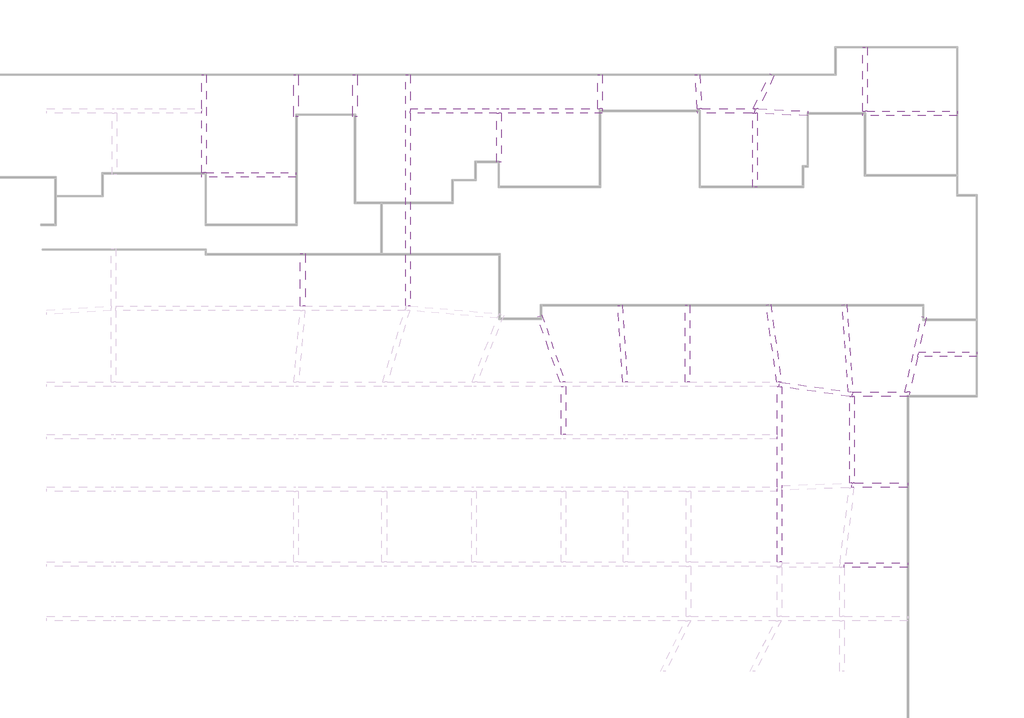
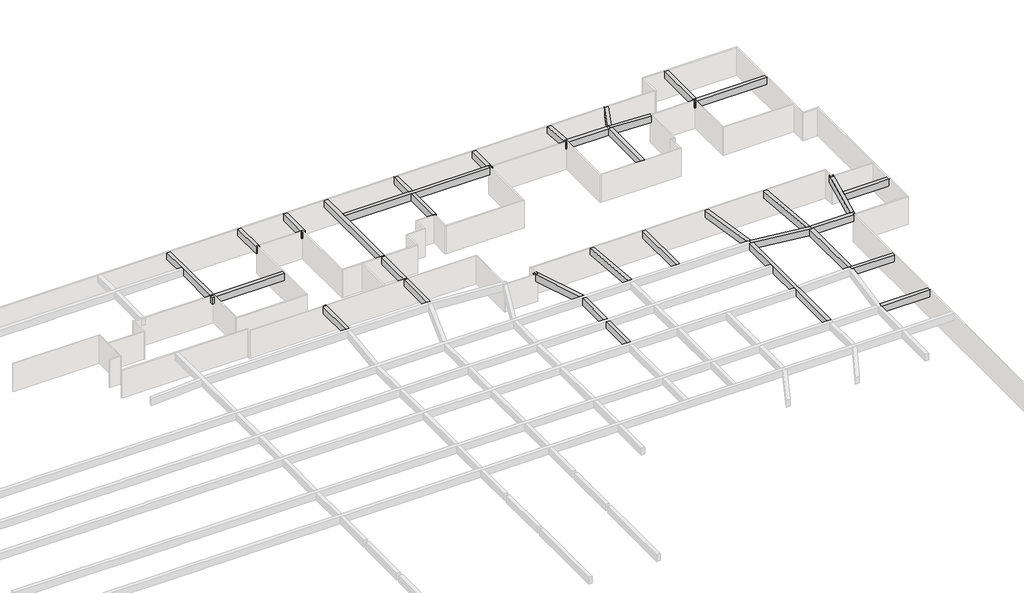
# One storey, part 45 of 45: 30 beams.
"""IFC4 building model written with IfcOpenShell, lengths in millimetres."""

import ifcopenshell
import ifcopenshell.guid

model = None  # the IFC model being written
_history = None  # IfcOwnerHistory: only IFC2X3 demands one
_inside = {}  # id of a spatial element -> (the spatial element, [elements in it])
_under = {}  # id of a project, library or spatial element -> (it, [spatial elements below it])
_declared = {}  # id of a project -> (the project, [libraries it declares])
_typed = {}  # id of a type object -> (the type object, [elements of that type])
_made_of = {}  # id of a material, layer set ... -> (it, [elements and type objects made of it])


def new_model(schema):
    """Start an empty IFC model of exactly this schema.

    Asked for "IFC4X3", IfcOpenShell would pick the latest addendum, in which some entities
    have other attributes; the version numbers below select the first issue.
    IFC2X3 requires an IfcOwnerHistory on every rooted entity: one is made here for all.
    """
    global model, _history
    if schema == "IFC4X3":
        model = ifcopenshell.file(schema_version=(4, 3, 0, 0))
    else:
        model = ifcopenshell.file(schema=schema)
    _inside.clear()
    _under.clear()
    _declared.clear()
    _typed.clear()
    _made_of.clear()
    _history = None
    if model.schema == "IFC2X3":
        org = make("IfcOrganization", Name="unknown")
        user = make(
            "IfcPersonAndOrganization",
            ThePerson=make("IfcPerson", FamilyName="unknown"),
            TheOrganization=org,
        )
        app = make(
            "IfcApplication",
            ApplicationDeveloper=org,
            Version="unknown",
            ApplicationFullName="unknown",
            ApplicationIdentifier="unknown",
        )
        _history = make(
            "IfcOwnerHistory",
            OwningUser=user,
            OwningApplication=app,
            ChangeAction="ADDED",
            CreationDate=0,
        )
    return model


def make(cls, **values):
    """One entity of the class cls with the attributes given. An attribute that is None is left unset."""
    return model.create_entity(
        cls, **{name: value for name, value in values.items() if value is not None}
    )


def rooted(cls, **values):
    """An entity with a GlobalId (a new one), such as an element, a storey or a relation."""
    return make(cls, GlobalId=ifcopenshell.guid.new(), OwnerHistory=_history, **values)


def si_unit(unit_type, name, prefix=None):
    """IfcSIUnit, for example si_unit("LENGTHUNIT", "METRE", prefix="MILLI")."""
    return make("IfcSIUnit", UnitType=unit_type, Prefix=prefix, Name=name)


def assignment(units):
    """IfcUnitAssignment: the units of a project."""
    return None if units is None else make("IfcUnitAssignment", Units=units)


def point(xyz):
    """IfcCartesianPoint."""
    return None if xyz is None else make("IfcCartesianPoint", Coordinates=xyz)


def direction(xyz):
    """IfcDirection."""
    return None if xyz is None else make("IfcDirection", DirectionRatios=xyz)


def frame(location, z_axis=None, x_axis=None):
    """IfcAxis2Placement3D, a coordinate frame: its origin and axes. An axis left out is left unset."""
    return make(
        "IfcAxis2Placement3D",
        Location=point(location),
        Axis=direction(z_axis),
        RefDirection=direction(x_axis),
    )


def origin():
    """The frame at (0, 0, 0) with its axes left unset."""
    return frame((0.0, 0.0, 0.0))


def place(relative_to, where):
    """IfcLocalPlacement: puts the frame where relative to a parent placement (None: the world)."""
    return make(
        "IfcLocalPlacement", PlacementRelTo=relative_to, RelativePlacement=where
    )


def context(
    kind, dimensions, precision=None, world=None, true_north=None, identifier=None
):
    """IfcGeometricRepresentationContext, for example the 3D "Model" context."""
    return make(
        "IfcGeometricRepresentationContext",
        ContextIdentifier=identifier,
        ContextType=kind,
        CoordinateSpaceDimension=dimensions,
        Precision=precision,
        WorldCoordinateSystem=world,
        TrueNorth=true_north,
    )


def project(units=None, contexts=None):
    """IfcProject with its units and contexts."""
    return rooted(
        "IfcProject",
        Name="project",
        RepresentationContexts=contexts,
        UnitsInContext=assignment(units),
    )


def spatial(cls, under=None, at=None, **own):
    """A site, building, storey or space (cls), placed at a placement, below another one or the project."""
    s = rooted(cls, ObjectPlacement=at, **own)
    if under is not None:
        _under.setdefault(under.id(), (under, []))[1].append(s)
    return s


def polyline(points):
    """IfcPolyline through the points."""
    return make("IfcPolyline", Points=[point(p) for p in points])


def outline(outer, holes=None, kind="AREA"):
    """IfcArbitraryClosedProfileDef: a profile drawn as a closed curve; with holes, ...WithVoids."""
    if holes is None:
        return make("IfcArbitraryClosedProfileDef", ProfileType=kind, OuterCurve=outer)
    return make(
        "IfcArbitraryProfileDefWithVoids",
        ProfileType=kind,
        OuterCurve=outer,
        InnerCurves=holes,
    )


def extrude(swept, where, along, depth):
    """IfcExtrudedAreaSolid: the profile swept, set in the frame where, extruded along a direction by depth."""
    return make(
        "IfcExtrudedAreaSolid",
        SweptArea=swept,
        Position=where,
        ExtrudedDirection=direction(along),
        Depth=depth,
    )


def faces_of(points, faces, orient=None, outer=None):
    """IfcFace entities. A face is a list of loops; a loop is a list of indices into points, from 0.

    orient and outer hold one flag for each loop. By default every Orientation is true, the
    first loop of a face is its IfcFaceOuterBound and the others are IfcFaceBound.
    """
    made = []
    for i, loops in enumerate(faces):
        bounds = []
        for j, loop in enumerate(loops):
            is_outer = j == 0 if outer is None else outer[i][j]
            bounds.append(
                make(
                    "IfcFaceOuterBound" if is_outer else "IfcFaceBound",
                    Bound=make("IfcPolyLoop", Polygon=[points[k] for k in loop]),
                    Orientation=True if orient is None else orient[i][j],
                )
            )
        made.append(make("IfcFace", Bounds=bounds))
    return made


def faceted_brep(points, faces, orient=None, outer=None, voids=None):
    """IfcFacetedBrep: a solid bounded by flat faces; with voids (closed shells), ...WithVoids."""
    shared = [point(p) for p in points]
    hull = make("IfcClosedShell", CfsFaces=faces_of(shared, faces, orient, outer))
    if voids is None:
        return make("IfcFacetedBrep", Outer=hull)
    return make(
        "IfcFacetedBrepWithVoids",
        Outer=hull,
        Voids=[
            make(cls, CfsFaces=faces_of(shared, fs, o, b)) for cls, fs, o, b in voids
        ],
    )


def shape(context_of_items, identifier, shape_type, items):
    """IfcShapeRepresentation: the items that make up one representation, for example the "Body"."""
    return make(
        "IfcShapeRepresentation",
        ContextOfItems=context_of_items,
        RepresentationIdentifier=identifier,
        RepresentationType=shape_type,
        Items=items,
    )


def source(mapping_origin, context_of_items, identifier, shape_type, items):
    """IfcRepresentationMap: a shape defined once, which mapped items show again and again."""
    return make(
        "IfcRepresentationMap",
        MappingOrigin=mapping_origin,
        MappedRepresentation=shape(context_of_items, identifier, shape_type, items),
    )


def transform(
    local_origin,
    x_axis=None,
    y_axis=None,
    z_axis=None,
    scale=None,
    scale2=None,
    scale3=None,
    uniform=True,
):
    """IfcCartesianTransformationOperator3D, or its non-uniform kind. x_axis, y_axis, z_axis: its Axis1, 2, 3."""
    if uniform:
        return make(
            "IfcCartesianTransformationOperator3D",
            Axis1=direction(x_axis),
            Axis2=direction(y_axis),
            LocalOrigin=point(local_origin),
            Scale=scale,
            Axis3=direction(z_axis),
        )
    return make(
        "IfcCartesianTransformationOperator3DnonUniform",
        Axis1=direction(x_axis),
        Axis2=direction(y_axis),
        LocalOrigin=point(local_origin),
        Scale=scale,
        Axis3=direction(z_axis),
        Scale2=scale2,
        Scale3=scale3,
    )


def mapped(mapping_source, mapping_target):
    """IfcMappedItem: shows the shape of a source again, moved by a transform."""
    return make(
        "IfcMappedItem", MappingSource=mapping_source, MappingTarget=mapping_target
    )


def made_of(thing, what):
    """Note that an element or type object is made of a material, layer set ...; save() writes the relation."""
    if what is not None:
        _made_of.setdefault(what.id(), (what, []))[1].append(thing)
    return thing


def element(
    cls,
    number,
    at=None,
    inside=None,
    cuts=None,
    type_object=None,
    material=None,
    context=None,
    identifier="Body",
    shape_type=None,
    held_by="IfcProductDefinitionShape",
    body=None,
    shapes=None,
    **own,
):
    """One element of the class cls, such as IfcWall. Its Tag is "e" and its number.

    at: its placement. inside: the storey or other place that contains it. cuts: it is an
    opening in that element (IfcRelVoidsElement). A single representation is given by context,
    identifier, shape_type and body (its items); several are given by shapes. held_by: the class
    of the entity that holds the representations. save() writes the other relations.
    """
    e = rooted(cls, Tag="e%d" % number, ObjectPlacement=at, **own)
    if body is not None:
        shapes = [shape(context, identifier, shape_type, body)]
    if shapes is not None:
        e.Representation = make(held_by, Representations=shapes)
    if inside is not None:
        _inside.setdefault(inside.id(), (inside, []))[1].append(e)
    if cuts is not None:
        rooted(
            "IfcRelVoidsElement", RelatingBuildingElement=cuts, RelatedOpeningElement=e
        )
    if type_object is not None:
        _typed.setdefault(type_object.id(), (type_object, []))[1].append(e)
    return made_of(e, material)


def aggregate(whole, parts):
    """IfcRelAggregates: a whole, such as a stair, and the parts it consists of."""
    return rooted("IfcRelAggregates", RelatingObject=whole, RelatedObjects=parts)


def save(model, path):
    """Write the relations noted so far, then the file.

    IfcRelAggregates (storeys below a building ...), IfcRelContainedInSpatialStructure (elements
    in a storey), IfcRelDefinesByType, IfcRelAssociatesMaterial and IfcRelDeclares: one each for
    every whole, place, type object, material and project.
    """
    for whole, parts in _under.values():
        aggregate(whole, parts)
    for where, things in _inside.values():
        rooted(
            "IfcRelContainedInSpatialStructure",
            RelatedElements=things,
            RelatingStructure=where,
        )
    for kind, things in _typed.values():
        rooted("IfcRelDefinesByType", RelatedObjects=things, RelatingType=kind)
    for what, things in _made_of.values():
        rooted("IfcRelAssociatesMaterial", RelatedObjects=things, RelatingMaterial=what)
    for by, libraries in _declared.values():
        rooted("IfcRelDeclares", RelatingContext=by, RelatedDefinitions=libraries)
    model.write(path)


def kl_beam_c459b6d2(model_context):
    return source(origin(), model_context, "Body", "SweptSolid", [
        extrude(outline(polyline([(1817.0, 200.0), (1817.0, -200.0), (-1817.0, -200.0), (-1817.0, 200.0), (1817.0, 200.0)])), frame((0.0, 0.0, -400.0), z_axis=(0.0, 0.0, 1.0), x_axis=(1.0, 0.0, 0.0)), (0.0, 0.0, 1.0), 800.0),
    ])


def kl_beam_000e6cef(model_context):
    return source(origin(), model_context, "Body", "SweptSolid", [
        extrude(outline(polyline([(1827.5, 200.0), (1827.5, -200.0), (-1827.5, -200.0), (-1827.5, 200.0), (1827.5, 200.0)])), frame((0.0, 0.0, -400.0), z_axis=(0.0, 0.0, 1.0), x_axis=(1.0, 0.0, 0.0)), (0.0, 0.0, 1.0), 800.0),
    ])


model = new_model("IFC4")

# Units and contexts
model_context = context("Model", 3, world=origin())
ifc_project = project(units=[si_unit("LENGTHUNIT", "METRE", prefix="MILLI")], contexts=[model_context])

# Site, building, storey
site = spatial("IfcSite", under=ifc_project)
building = spatial("IfcBuilding", under=site)
storey = spatial("IfcBuildingStorey", under=building, Name="户型图", Elevation=0.0)

# Beams
placement = place(None, origin())
element("IfcBeam", 1, ObjectType="混凝土 - 矩形梁 : KL_beam", at=placement, inside=storey, context=model_context, shape_type="SweptSolid", body=[
    extrude(outline(polyline([(10558.170888, 195578.568213), (10958.170888, 195578.568213), (10958.170888, 191034.1392013), (10558.170888, 191034.1392013), (10558.170888, 195578.568213)])), frame((0.0, 0.0, 2500.0), z_axis=(0.0, 0.0, 1.0), x_axis=(1.0, 0.0, 0.0)), (0.0, 0.0, 1.0), 800.0),
])
element("IfcBeam", 2, ObjectType="混凝土 - 矩形梁 : KL_beam", at=placement, inside=storey, context=model_context, shape_type="SweptSolid", body=[
    extrude(outline(polyline([(38177.3384091, 191063.5546545), (38576.3640292, 191091.457244), (39044.6739052, 184394.3140025), (38643.697146, 184394.3140025), (38177.3384091, 191063.5546545)])), frame((0.0, 0.0, 2500.0), z_axis=(0.0, 0.0, 1.0), x_axis=(1.0, 0.0, 0.0)), (0.0, 0.0, 1.0), 800.0),
])
element("IfcBeam", 3, ObjectType="混凝土 - 矩形梁 : KL_beam", at=placement, inside=storey, context=model_context, shape_type="SweptSolid", body=[
    extrude(outline(polyline([(44058.170888, 191094.3140025), (44458.170888, 191094.3140025), (44458.170888, 184394.3140025), (44058.170888, 184394.3140025), (44058.170888, 191094.3140025)])), frame((0.0, 0.0, 2500.0), z_axis=(0.0, 0.0, 1.0), x_axis=(1.0, 0.0, 0.0)), (0.0, 0.0, 1.0), 800.0),
])
element("IfcBeam", 4, ObjectType="混凝土 - 矩形梁 : KL_beam", at=placement, inside=storey, context=model_context, shape_type="Brep", body=[
    faceted_brep([(58656.8908977, 183499.9137112, 3300.0), (58251.9343991, 183556.8266355, 3300.0), (52455.9955059, 184371.3927255, 3300.0), (52292.9021454, 184394.3140025, 3300.0), (52264.9314206, 183994.3140025, 3300.0), (52492.6053307, 183962.3165211, 3300.0), (58384.2248716, 183134.3033931, 3300.0), (58601.2216573, 183103.8064837, 3300.0), (58604.1159054, 183124.4001284, 3300.0), (52264.9314206, 183994.3140025, 2500.0), (52492.6053307, 183962.3165211, 2500.0), (58384.2248716, 183134.3033931, 2500.0), (58601.2216573, 183103.8064837, 2500.0), (52292.9021454, 184394.3140025, 2500.0), (52455.9955059, 184371.3927255, 2500.0), (58251.9343991, 183556.8266355, 2500.0), (58656.8908977, 183499.9137112, 2500.0), (58604.1159054, 183124.4001284, 2500.0)], [[[0, 1, 2, 3, 4, 5, 6, 7, 8]], [[7, 6, 5, 4, 9, 10, 11, 12]], [[12, 11, 10, 9, 13, 14, 15, 16, 17]], [[3, 2, 1, 0, 16, 15, 14, 13]], [[3, 13, 9, 4]], [[0, 8, 7, 12, 17, 16]]]),
])
element("IfcBeam", 5, ObjectType="混凝土 - 矩形梁 : KL_beam", at=placement, inside=storey, context=model_context, shape_type="SweptSolid", body=[
    extrude(outline(polyline([(51106.6514625, 191098.3558635), (51502.75869, 191154.0251039), (52455.9955059, 184371.3927255), (52292.9021454, 184394.3140025), (52048.8431015, 184394.3140025), (51106.6514625, 191098.3558635)])), frame((0.0, 0.0, 2500.0), z_axis=(0.0, 0.0, 1.0), x_axis=(1.0, 0.0, 0.0)), (0.0, 0.0, 1.0), 800.0),
])
element("IfcBeam", 6, ObjectType="混凝土 - 矩形梁 : KL_beam", at=placement, inside=storey, context=model_context, shape_type="Brep", body=[
    faceted_brep([(58122.1746543, 191146.7122502, 3300.0), (58122.1746543, 191146.7122502, 2500.0), (57723.1490342, 191118.8096607, 2500.0), (57723.1490342, 191118.8096607, 3300.0), (58251.9343991, 183556.8266355, 3300.0), (58656.8908977, 183499.9137112, 3300.0), (58655.1786406, 183524.4001284, 3300.0), (58251.9343991, 183556.8266355, 2500.0), (58655.1786406, 183524.4001284, 2500.0), (58656.8908977, 183499.9137112, 2500.0)], [[[0, 1, 2, 3]], [[0, 3, 4, 5, 6]], [[3, 2, 7, 4]], [[2, 1, 8, 9, 7]], [[1, 0, 6, 5, 9, 8]], [[5, 4, 7, 9]]]),
])
element("IfcBeam", 7, ObjectType="混凝土 - 矩形梁 : KL_beam", at=placement, inside=storey, context=model_context, shape_type="Brep", body=[
    faceted_brep([(58656.8908977, 183499.9137112, 3300.0), (58604.1159054, 183124.4001284, 3300.0), (58784.2248716, 183124.4001284, 3300.0), (63529.491463, 183124.4001284, 3300.0), (63617.407341, 183524.4001284, 3300.0), (63207.8597838, 183524.4001284, 3300.0), (58655.1786406, 183524.4001284, 3300.0), (58604.1159054, 183124.4001284, 2500.0), (58784.2248716, 183124.4001284, 2500.0), (63529.491463, 183124.4001284, 2500.0), (58656.8908977, 183499.9137112, 2500.0), (58655.1786406, 183524.4001284, 2500.0), (63207.8597838, 183524.4001284, 2500.0), (63617.407341, 183524.4001284, 2500.0)], [[[0, 1, 2, 3, 4, 5, 6]], [[1, 7, 8, 9, 3, 2]], [[7, 10, 11, 12, 13, 9, 8]], [[4, 13, 12, 11, 6, 5]], [[1, 0, 10, 7]], [[0, 6, 11, 10]], [[4, 3, 9, 13]]]),
])
element("IfcBeam", 8, ObjectType="混凝土 - 矩形梁 : KL_beam", at=placement, inside=storey, context=model_context, shape_type="Brep", body=[
    faceted_brep([(65041.3670071, 190003.1373024, 3300.0), (65041.3670071, 190003.1373024, 2500.0), (64650.6919873, 190089.0036458, 2500.0), (64650.6919873, 190089.0036458, 3300.0), (63207.8597838, 183524.4001284, 3300.0), (63617.407341, 183524.4001284, 3300.0), (64298.4480041, 186623.0015609, 3300.0), (64386.363882, 187023.0015609, 3300.0), (63207.8597838, 183524.4001284, 2500.0), (64386.363882, 187023.0015609, 2500.0), (64298.4480041, 186623.0015609, 2500.0), (63617.407341, 183524.4001284, 2500.0)], [[[0, 1, 2, 3]], [[0, 3, 4, 5, 6, 7]], [[3, 2, 8, 4]], [[2, 1, 9, 10, 11, 8]], [[1, 0, 7, 6, 5, 11, 10, 9]], [[5, 4, 8, 11]]]),
])
element("IfcBeam", 9, ObjectType="混凝土 - 矩形梁 : KL_beam", at=placement, inside=storey, context=model_context, shape_type="SweptSolid", body=[
    extrude(outline(polyline([(69459.055254, 187023.0015609), (69459.055254, 186623.0015609), (64298.4480041, 186623.0015609), (64386.363882, 187023.0015609), (69459.055254, 187023.0015609)])), frame((0.0, 0.0, 2500.0), z_axis=(0.0, 0.0, 1.0), x_axis=(1.0, 0.0, 0.0)), (0.0, 0.0, 1.0), 800.0),
])
element("IfcBeam", 10, ObjectType="混凝土 - 矩形梁 : KL_beam", at=placement, inside=storey, context=model_context, shape_type="SweptSolid", body=[
    extrude(outline(polyline([(33258.170888, 183994.3140025), (33658.170888, 183994.3140025), (33658.170888, 179811.4368869), (33258.170888, 179811.4368869), (33258.170888, 183994.3140025)])), frame((0.0, 0.0, 2500.0), z_axis=(0.0, 0.0, 1.0), x_axis=(1.0, 0.0, 0.0)), (0.0, 0.0, 1.0), 800.0),
    extrude(outline(polyline([(33658.170888, 175259.2955299), (33258.170888, 175259.2955299), (33258.170888, 179411.4368869), (33658.170888, 179411.4368869), (33658.170888, 175259.2955299)])), frame((0.0, 0.0, 2500.0), z_axis=(0.0, 0.0, 1.0), x_axis=(1.0, 0.0, 0.0)), (0.0, 0.0, 1.0), 800.0),
])
element("IfcBeam", 11, ObjectType="混凝土 - 矩形梁 : KL_beam", at=placement, inside=storey, context=model_context, shape_type="SweptSolid", body=[
    extrude(outline(polyline([(31217.9877998, 190085.9673979), (31596.19523, 190216.1946597), (33600.8295016, 184394.3140025), (33177.7812291, 184394.3140025), (31217.9877998, 190085.9673979)])), frame((0.0, 0.0, 2500.0), z_axis=(0.0, 0.0, 1.0), x_axis=(1.0, 0.0, 0.0)), (0.0, 0.0, 1.0), 800.0),
])
element("IfcBeam", 12, ObjectType="混凝土 - 矩形梁 : KL_beam", at=placement, inside=storey, context=model_context, shape_type="Brep", body=[
    faceted_brep([(19735.6474887, 211171.5634374, 3300.0), (20135.6474887, 211171.5634374, 3300.0), (20135.6474887, 211171.5634374, 2500.0), (19735.6474887, 211171.5634374, 2500.0), (19735.6474887, 191052.4009015, 3300.0), (20135.6474887, 191017.4054361, 3300.0), (20135.6474887, 207811.9876735, 3300.0), (20135.6474887, 208211.9876735, 3300.0), (20135.6474887, 191017.4054361, 2500.0), (20135.6474887, 207811.9876735, 2500.0), (20135.6474887, 208211.9876735, 2500.0), (19735.6474887, 191052.4009015, 2500.0)], [[[0, 1, 2, 3]], [[1, 0, 4, 5, 6, 7]], [[2, 1, 7, 6, 5, 8, 9, 10]], [[3, 2, 10, 9, 8, 11]], [[0, 3, 11, 4]], [[5, 4, 11, 8]]]),
])
element("IfcBeam", 13, ObjectType="混凝土 - 矩形梁 : KL_beam", at=placement, inside=storey, context=model_context, shape_type="Brep", body=[
    faceted_brep([(36835.6474887, 207811.9876735, 3300.0), (36835.6474887, 208211.9876735, 3300.0), (36435.6474887, 208211.9876735, 3300.0), (28035.6474887, 208211.9876735, 3300.0), (27635.6474887, 208211.9876735, 3300.0), (20135.6474887, 208211.9876735, 3300.0), (20135.6474887, 207811.9876735, 3300.0), (27635.6474887, 207811.9876735, 3300.0), (28035.6474887, 207811.9876735, 3300.0), (36835.6474887, 207811.9876735, 2500.0), (20135.6474887, 207811.9876735, 2500.0), (27635.6474887, 207811.9876735, 2500.0), (28035.6474887, 207811.9876735, 2500.0), (36835.6474887, 208211.9876735, 2500.0), (20135.6474887, 208211.9876735, 2500.0), (27635.6474887, 208211.9876735, 2500.0), (28035.6474887, 208211.9876735, 2500.0), (36435.6474887, 208211.9876735, 2500.0)], [[[0, 1, 2, 3, 4, 5, 6, 7, 8]], [[9, 0, 8, 7, 6, 10, 11, 12]], [[13, 9, 12, 11, 10, 14, 15, 16, 17]], [[1, 13, 17, 16, 15, 14, 5, 4, 3, 2]], [[6, 5, 14, 10]], [[1, 0, 9, 13]]]),
])
element("IfcBeam", 14, ObjectType="混凝土 - 矩形梁 : KL_beam", at=placement, inside=storey, context=model_context, shape_type="SweptSolid", body=[
    extrude(outline(polyline([(36435.6474887, 211171.9876735), (36835.6474887, 211171.9876735), (36835.6474887, 208211.9876735), (36435.6474887, 208211.9876735), (36435.6474887, 211171.9876735)])), frame((0.0, 0.0, 2500.0), z_axis=(0.0, 0.0, 1.0), x_axis=(1.0, 0.0, 0.0)), (0.0, 0.0, 1.0), 800.0),
])
element("IfcBeam", 15, ObjectType="混凝土 - 矩形梁 : KL_beam", at=placement, inside=storey, context=model_context, shape_type="SweptSolid", body=[
    extrude(outline(polyline([(28035.6474887, 203571.9876735), (27635.6474887, 203571.9876735), (27635.6474887, 207811.9876735), (28035.6474887, 207811.9876735), (28035.6474887, 203571.9876735)])), frame((0.0, 0.0, 2500.0), z_axis=(0.0, 0.0, 1.0), x_axis=(1.0, 0.0, 0.0)), (0.0, 0.0, 1.0), 800.0),
    extrude(outline(polyline([(27635.6474887, 211171.9876735), (28035.6474887, 211171.9876735), (28035.6474887, 208211.9876735), (27635.6474887, 208211.9876735), (27635.6474887, 211171.9876735)])), frame((0.0, 0.0, 2500.0), z_axis=(0.0, 0.0, 1.0), x_axis=(1.0, 0.0, 0.0)), (0.0, 0.0, 1.0), 800.0),
])
element("IfcBeam", 16, ObjectType="混凝土 - 矩形梁 : KL_beam", at=placement, inside=storey, context=model_context, shape_type="Brep", body=[
    faceted_brep([(10170.4764011, 202651.2886433, 3300.0), (10170.4764011, 202251.2886433, 3300.0), (10170.4764011, 202251.2886433, 2500.0), (10170.4764011, 202651.2886433, 2500.0), (2351.1462183, 202651.2886433, 3300.0), (1951.1462183, 202651.2886433, 3300.0), (1951.1462183, 202251.2886433, 3300.0), (1951.1462183, 202251.2886433, 2500.0), (1951.1462183, 202651.2886433, 2500.0), (2351.1462183, 202651.2886433, 2500.0)], [[[0, 1, 2, 3]], [[1, 0, 4, 5, 6]], [[2, 1, 6, 7]], [[3, 2, 7, 8, 9]], [[0, 3, 9, 8, 5, 4]], [[6, 5, 8, 7]]]),
])
element("IfcBeam", 17, ObjectType="混凝土 - 矩形梁 : KL_beam", at=placement, inside=storey, context=model_context, shape_type="Brep", body=[
    faceted_brep([(1951.1462183, 211171.6381584, 3300.0), (2351.1462183, 211171.6381584, 3300.0), (2351.1462183, 211171.6381584, 2500.0), (1951.1462183, 211171.6381584, 2500.0), (1951.1462183, 208211.9876735, 3300.0), (1951.1462183, 207811.9876735, 3300.0), (1951.1462183, 202651.2886433, 3300.0), (2351.1462183, 202651.2886433, 3300.0), (2351.1462183, 202651.2886433, 2500.0), (1951.1462183, 202651.2886433, 2500.0), (1951.1462183, 207811.9876735, 2500.0), (1951.1462183, 208211.9876735, 2500.0)], [[[0, 1, 2, 3]], [[1, 0, 4, 5, 6, 7]], [[2, 1, 7, 8]], [[3, 2, 8, 9, 10, 11]], [[0, 3, 11, 10, 9, 6, 5, 4]], [[7, 6, 9, 8]]]),
])
element("IfcBeam", 18, ObjectType="混凝土 - 矩形梁 : KL_beam", at=placement, inside=storey, context=model_context, shape_type="Brep", body=[
    faceted_brep([(52092.6053307, 168716.2365071, 3300.0), (52492.6053307, 168716.2365071, 3300.0), (52492.6053307, 174976.174955, 3300.0), (52492.6053307, 175376.4187727, 3300.0), (52492.6053307, 183962.3165211, 3300.0), (52264.9314206, 183994.3140025, 3300.0), (52092.6053307, 183994.3140025, 3300.0), (52092.6053307, 179811.4368869, 3300.0), (52092.6053307, 179411.4368869, 3300.0), (52092.6053307, 175259.2955299, 3300.0), (52092.6053307, 174859.2955299, 3300.0), (52492.6053307, 168716.2365071, 2500.0), (52492.6053307, 174976.174955, 2500.0), (52492.6053307, 175376.4187727, 2500.0), (52492.6053307, 183962.3165211, 2500.0), (52092.6053307, 168716.2365071, 2500.0), (52092.6053307, 174859.2955299, 2500.0), (52092.6053307, 175259.2955299, 2500.0), (52092.6053307, 179411.4368869, 2500.0), (52092.6053307, 179811.4368869, 2500.0), (52092.6053307, 183994.3140025, 2500.0), (52264.9314206, 183994.3140025, 2500.0)], [[[0, 1, 2, 3, 4, 5, 6, 7, 8, 9, 10]], [[1, 11, 12, 13, 14, 4, 3, 2]], [[11, 15, 16, 17, 18, 19, 20, 21, 14, 13, 12]], [[15, 0, 10, 9, 8, 7, 6, 20, 19, 18, 17, 16]], [[1, 0, 15, 11]], [[5, 4, 14, 21]], [[6, 5, 21, 20]]]),
])
element("IfcBeam", 19, ObjectType="混凝土 - 矩形梁 : KL_beam", at=placement, inside=storey, context=model_context, shape_type="Brep", body=[
    faceted_brep([(63459.2248716, 175589.0120542, 3300.0), (63459.2248716, 175189.0120542, 3300.0), (63459.2248716, 175189.0120542, 2500.0), (63459.2248716, 175589.0120542, 2500.0), (58784.2248716, 175589.0120542, 3300.0), (58580.4803867, 175589.0120542, 3300.0), (58587.4624127, 175189.0120542, 3300.0), (58760.8164767, 175189.0120542, 3300.0), (58587.4624127, 175189.0120542, 2500.0), (58760.8164767, 175189.0120542, 2500.0), (58580.4803867, 175589.0120542, 2500.0), (58784.2248716, 175589.0120542, 2500.0)], [[[0, 1, 2, 3]], [[1, 0, 4, 5, 6, 7]], [[2, 1, 7, 6, 8, 9]], [[3, 2, 9, 8, 10, 11]], [[0, 3, 11, 10, 5, 4]], [[5, 10, 8, 6]]]),
])
element("IfcBeam", 20, ObjectType="混凝土 - 矩形梁 : KL_beam", at=placement, inside=storey, context=model_context, shape_type="SweptSolid", body=[
    extrude(outline(polyline([(58784.2248716, 175589.0120542), (58580.4803867, 175589.0120542), (58384.2248716, 175582.1586606), (58384.2248716, 183134.3033931), (58601.2216573, 183103.8064837), (58604.1159054, 183124.4001284), (58784.2248716, 183124.4001284), (58784.2248716, 175589.0120542)])), frame((0.0, 0.0, 2500.0), z_axis=(0.0, 0.0, 1.0), x_axis=(1.0, 0.0, 0.0)), (0.0, 0.0, 1.0), 800.0),
])
element("IfcBeam", 21, ObjectType="混凝土 - 矩形梁 : KL_beam", at=placement, inside=storey, context=model_context, shape_type="Brep", body=[
    faceted_brep([(63430.7855894, 168641.1854865, 3300.0), (63430.7855894, 168241.1854865, 3300.0), (63430.7855894, 168241.1854865, 2500.0), (63430.7855894, 168641.1854865, 2500.0), (57956.8444667, 168641.1854865, 3300.0), (57907.7306423, 168241.1854865, 3300.0), (57931.1254195, 168241.1854865, 3300.0), (57907.7306423, 168241.1854865, 2500.0), (57931.1254195, 168241.1854865, 2500.0), (57956.8444667, 168641.1854865, 2500.0)], [[[0, 1, 2, 3]], [[1, 0, 4, 5, 6]], [[2, 1, 6, 5, 7, 8]], [[3, 2, 8, 7, 9]], [[0, 3, 9, 4]], [[5, 4, 9, 7]]]),
])
element("IfcBeam", 22, ObjectType="混凝土 - 矩形梁 : KL_beam", at=placement, inside=storey, context=model_context, shape_type="Brep", body=[
    faceted_brep([(50130.8671853, 207811.9876735, 3300.0), (50140.4277921, 208211.9876735, 3300.0), (50008.2380177, 208211.9876735, 3300.0), (45522.1505059, 208211.9876735, 3300.0), (45121.1737467, 208211.9876735, 3300.0), (45149.1444714, 207811.9876735, 3300.0), (49935.6474887, 207811.9876735, 3300.0), (50130.8671853, 207811.9876735, 2500.0), (45149.1444714, 207811.9876735, 2500.0), (49935.6474887, 207811.9876735, 2500.0), (50140.4277921, 208211.9876735, 2500.0), (45121.1737467, 208211.9876735, 2500.0), (45522.1505059, 208211.9876735, 2500.0), (50008.2380177, 208211.9876735, 2500.0)], [[[0, 1, 2, 3, 4, 5, 6]], [[7, 0, 6, 5, 8, 9]], [[10, 7, 9, 8, 11, 12, 13]], [[1, 10, 13, 12, 11, 4, 3, 2]], [[1, 0, 7, 10]], [[5, 4, 11, 8]]]),
])
element("IfcBeam", 23, ObjectType="混凝土 - 矩形梁 : KL_beam", at=placement, inside=storey, context=model_context, shape_type="Brep", body=[
    faceted_brep([(54745.0733828, 207991.7458244, 3300.0), (54725.9630867, 207592.2025894, 3300.0), (54725.9630867, 207592.2025894, 2500.0), (54745.0733828, 207991.7458244, 2500.0), (50442.844192, 208197.5229887, 3300.0), (50140.4277921, 208211.9876735, 3300.0), (50130.8671853, 207811.9876735, 3300.0), (50335.6474887, 207802.1929582, 3300.0), (50130.8671853, 207811.9876735, 2500.0), (50335.6474887, 207802.1929582, 2500.0), (50140.4277921, 208211.9876735, 2500.0), (50442.844192, 208197.5229887, 2500.0)], [[[0, 1, 2, 3]], [[1, 0, 4, 5, 6, 7]], [[2, 1, 7, 6, 8, 9]], [[3, 2, 9, 8, 10, 11]], [[0, 3, 11, 10, 5, 4]], [[5, 10, 8, 6]]]),
])
element("IfcBeam", 24, ObjectType="混凝土 - 矩形梁 : KL_beam", at=placement, inside=storey, context=model_context, shape_type="SweptSolid", body=[
    extrude(outline(polyline([(50335.6474887, 201391.9778491), (49935.6474887, 201391.9778491), (49935.6474887, 207811.9876735), (50130.8671853, 207811.9876735), (50335.6474887, 207802.1929582), (50335.6474887, 201391.9778491)])), frame((0.0, 0.0, 2500.0), z_axis=(0.0, 0.0, 1.0), x_axis=(1.0, 0.0, 0.0)), (0.0, 0.0, 1.0), 800.0),
])
element("IfcBeam", 25, ObjectType="混凝土 - 矩形梁 : KL_beam", at=placement, inside=storey, context=model_context, shape_type="Brep", body=[
    faceted_brep([(67759.2706298, 207991.9680247, 3300.0), (67759.2706298, 207591.9680247, 3300.0), (67759.2706298, 207591.9680247, 2500.0), (67759.2706298, 207991.9680247, 2500.0), (59936.0629161, 207991.9680247, 3300.0), (59536.0629161, 207991.9680247, 3300.0), (59536.0629161, 207591.9680247, 3300.0), (59536.0629161, 207591.9680247, 2500.0), (59536.0629161, 207991.9680247, 2500.0), (59936.0629161, 207991.9680247, 2500.0)], [[[0, 1, 2, 3]], [[1, 0, 4, 5, 6]], [[2, 1, 6, 7]], [[3, 2, 7, 8, 9]], [[0, 3, 9, 8, 5, 4]], [[6, 5, 8, 7]]]),
])
element("IfcBeam", 26, ObjectType="混凝土 - 矩形梁 : KL_beam", at=placement, inside=storey, context=model_context, shape_type="SweptSolid", body=[
    extrude(outline(polyline([(59536.0629161, 213571.9778491), (59936.0629161, 213571.9778491), (59936.0629161, 207991.9680247), (59536.0629161, 207991.9680247), (59536.0629161, 213571.9778491)])), frame((0.0, 0.0, 2500.0), z_axis=(0.0, 0.0, 1.0), x_axis=(1.0, 0.0, 0.0)), (0.0, 0.0, 1.0), 800.0),
])
element("IfcBeam", 27, ObjectType="混凝土 - 矩形梁 : KL_beam", at=placement, inside=storey, context=model_context, shape_type="SweptSolid", body=[
    extrude(outline(polyline([(44915.1909396, 211157.6790524), (45314.2165597, 211185.5816419), (45522.1505059, 208211.9876735), (45121.1737467, 208211.9876735), (44915.1909396, 211157.6790524)])), frame((0.0, 0.0, 2500.0), z_axis=(0.0, 0.0, 1.0), x_axis=(1.0, 0.0, 0.0)), (0.0, 0.0, 1.0), 800.0),
])
element("IfcBeam", 28, ObjectType="混凝土 - 矩形梁 : KL_beam", at=placement, inside=storey, context=model_context, shape_type="SweptSolid", body=[
    extrude(outline(polyline([(51427.777952, 211256.2008865), (51790.3010668, 211087.1535818), (50442.844192, 208197.5229887), (50140.4277921, 208211.9876735), (50008.2380177, 208211.9876735), (51427.777952, 211256.2008865)])), frame((0.0, 0.0, 2500.0), z_axis=(0.0, 0.0, 1.0), x_axis=(1.0, 0.0, 0.0)), (0.0, 0.0, 1.0), 800.0),
])
kl_beam_shape = kl_beam_c459b6d2(model_context)
element("IfcBeam", 29, ObjectType="混凝土 - 矩形梁 : KL_beam", at=placement, inside=storey, context=model_context, shape_type="MappedRepresentation", body=[
    mapped(kl_beam_shape, transform((15316.9563477, 209354.6929907, 2900.0), x_axis=(0.0, 1.0, 0.0), y_axis=(-1.0, 0.0, 0.0), z_axis=(0.0, 0.0, 1.0))),
])
kl_beam_2_shape = kl_beam_000e6cef(model_context)
element("IfcBeam", 30, ObjectType="混凝土 - 矩形梁 : KL_beam", at=placement, inside=storey, context=model_context, shape_type="MappedRepresentation", body=[
    mapped(kl_beam_2_shape, transform((10170.8065839, 209344.0823727, 2900.0), x_axis=(0.0, 1.0, 0.0), y_axis=(-1.0, 0.0, 0.0), z_axis=(0.0, 0.0, 1.0))),
])

save(model, "model.ifc")

# Revit data of these elements
# Type "混凝土 - 矩形梁 : KL_beam"
#   Length [instance default] = 1524 mm
#   b = 400 mm
#   h = 800 mm
#   Structural Material [instance default] = 混凝土 - 现场浇注混凝土
#   Assembly Code = ""
# Elements 1, 2, 3, 4, 5, 6, 7, 8, 9, 10, 11, 12, 13, 14, 15, 16, 17, 18, 19, 20, 21, 22, 23, 24, 25, 26, 27, 28, 29, 30 (IfcBeam, "混凝土 - 矩形梁 : KL_beam")
#   Comments = ""
#   Structural Material = none
#   Phase Created = 新构造
# Materials
#   "混凝土 - 现场浇注混凝土": class "混凝土", colour RGB 192 192 192, transparency 0
